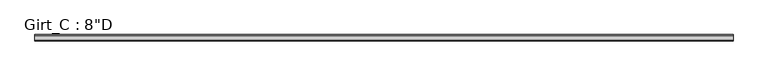
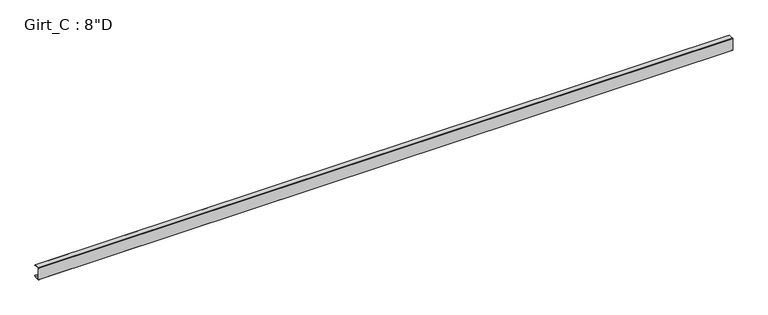
"""IFC4 building model written with IfcOpenShell, lengths in millimetres: beam geometry."""

import ifcopenshell
import ifcopenshell.guid

model = None  # the IFC model being written
_history = None  # IfcOwnerHistory: only IFC2X3 demands one
_inside = {}  # id of a spatial element -> (the spatial element, [elements in it])
_under = {}  # id of a project, library or spatial element -> (it, [spatial elements below it])
_declared = {}  # id of a project -> (the project, [libraries it declares])
_typed = {}  # id of a type object -> (the type object, [elements of that type])
_made_of = {}  # id of a material, layer set ... -> (it, [elements and type objects made of it])


def new_model(schema):
    """Start an empty IFC model of exactly this schema.

    Asked for "IFC4X3", IfcOpenShell would pick the latest addendum, in which some entities
    have other attributes; the version numbers below select the first issue.
    IFC2X3 requires an IfcOwnerHistory on every rooted entity: one is made here for all.
    """
    global model, _history
    if schema == "IFC4X3":
        model = ifcopenshell.file(schema_version=(4, 3, 0, 0))
    else:
        model = ifcopenshell.file(schema=schema)
    _inside.clear()
    _under.clear()
    _declared.clear()
    _typed.clear()
    _made_of.clear()
    _history = None
    if model.schema == "IFC2X3":
        org = make("IfcOrganization", Name="unknown")
        user = make(
            "IfcPersonAndOrganization",
            ThePerson=make("IfcPerson", FamilyName="unknown"),
            TheOrganization=org,
        )
        app = make(
            "IfcApplication",
            ApplicationDeveloper=org,
            Version="unknown",
            ApplicationFullName="unknown",
            ApplicationIdentifier="unknown",
        )
        _history = make(
            "IfcOwnerHistory",
            OwningUser=user,
            OwningApplication=app,
            ChangeAction="ADDED",
            CreationDate=0,
        )
    return model


def make(cls, **values):
    """One entity of the class cls with the attributes given. An attribute that is None is left unset."""
    return model.create_entity(
        cls, **{name: value for name, value in values.items() if value is not None}
    )


def rooted(cls, **values):
    """An entity with a GlobalId (a new one), such as an element, a storey or a relation."""
    return make(cls, GlobalId=ifcopenshell.guid.new(), OwnerHistory=_history, **values)


def si_unit(unit_type, name, prefix=None):
    """IfcSIUnit, for example si_unit("LENGTHUNIT", "METRE", prefix="MILLI")."""
    return make("IfcSIUnit", UnitType=unit_type, Prefix=prefix, Name=name)


def assignment(units):
    """IfcUnitAssignment: the units of a project."""
    return None if units is None else make("IfcUnitAssignment", Units=units)


def point(xyz):
    """IfcCartesianPoint."""
    return None if xyz is None else make("IfcCartesianPoint", Coordinates=xyz)


def direction(xyz):
    """IfcDirection."""
    return None if xyz is None else make("IfcDirection", DirectionRatios=xyz)


def frame(location, z_axis=None, x_axis=None):
    """IfcAxis2Placement3D, a coordinate frame: its origin and axes. An axis left out is left unset."""
    return make(
        "IfcAxis2Placement3D",
        Location=point(location),
        Axis=direction(z_axis),
        RefDirection=direction(x_axis),
    )


def frame_2d(location, x_axis=None):
    """IfcAxis2Placement2D, a coordinate frame in the plane: its origin and x axis."""
    return make(
        "IfcAxis2Placement2D", Location=point(location), RefDirection=direction(x_axis)
    )


def origin():
    """The frame at (0, 0, 0) with its axes left unset."""
    return frame((0.0, 0.0, 0.0))


def place(relative_to, where):
    """IfcLocalPlacement: puts the frame where relative to a parent placement (None: the world)."""
    return make(
        "IfcLocalPlacement", PlacementRelTo=relative_to, RelativePlacement=where
    )


def context(
    kind, dimensions, precision=None, world=None, true_north=None, identifier=None
):
    """IfcGeometricRepresentationContext, for example the 3D "Model" context."""
    return make(
        "IfcGeometricRepresentationContext",
        ContextIdentifier=identifier,
        ContextType=kind,
        CoordinateSpaceDimension=dimensions,
        Precision=precision,
        WorldCoordinateSystem=world,
        TrueNorth=true_north,
    )


def project(units=None, contexts=None):
    """IfcProject with its units and contexts."""
    return rooted(
        "IfcProject",
        Name="project",
        RepresentationContexts=contexts,
        UnitsInContext=assignment(units),
    )


def spatial(cls, under=None, at=None, **own):
    """A site, building, storey or space (cls), placed at a placement, below another one or the project."""
    s = rooted(cls, ObjectPlacement=at, **own)
    if under is not None:
        _under.setdefault(under.id(), (under, []))[1].append(s)
    return s


def polyline(points):
    """IfcPolyline through the points."""
    return make("IfcPolyline", Points=[point(p) for p in points])


def circle_curve(where, radius):
    """IfcCircle in the frame where."""
    return make("IfcCircle", Position=where, Radius=radius)


def trimmed(basis, trim1, trim2, sense, master):
    """IfcTrimmedCurve: the piece of a basis curve between two trims."""
    return make(
        "IfcTrimmedCurve",
        BasisCurve=basis,
        Trim1=trim1,
        Trim2=trim2,
        SenseAgreement=sense,
        MasterRepresentation=master,
    )


def segment(curve, same_sense, transition):
    """IfcCompositeCurveSegment."""
    return make(
        "IfcCompositeCurveSegment",
        Transition=transition,
        SameSense=same_sense,
        ParentCurve=curve,
    )


def composite_curve(segments, self_intersect=None):
    """IfcCompositeCurve: segments joined end to end."""
    return make("IfcCompositeCurve", Segments=segments, SelfIntersect=self_intersect)


def outline(outer, holes=None, kind="AREA"):
    """IfcArbitraryClosedProfileDef: a profile drawn as a closed curve; with holes, ...WithVoids."""
    if holes is None:
        return make("IfcArbitraryClosedProfileDef", ProfileType=kind, OuterCurve=outer)
    return make(
        "IfcArbitraryProfileDefWithVoids",
        ProfileType=kind,
        OuterCurve=outer,
        InnerCurves=holes,
    )


def extrude(swept, where, along, depth):
    """IfcExtrudedAreaSolid: the profile swept, set in the frame where, extruded along a direction by depth."""
    return make(
        "IfcExtrudedAreaSolid",
        SweptArea=swept,
        Position=where,
        ExtrudedDirection=direction(along),
        Depth=depth,
    )


def shape(context_of_items, identifier, shape_type, items):
    """IfcShapeRepresentation: the items that make up one representation, for example the "Body"."""
    return make(
        "IfcShapeRepresentation",
        ContextOfItems=context_of_items,
        RepresentationIdentifier=identifier,
        RepresentationType=shape_type,
        Items=items,
    )


def source(mapping_origin, context_of_items, identifier, shape_type, items):
    """IfcRepresentationMap: a shape defined once, which mapped items show again and again."""
    return make(
        "IfcRepresentationMap",
        MappingOrigin=mapping_origin,
        MappedRepresentation=shape(context_of_items, identifier, shape_type, items),
    )


def transform(
    local_origin,
    x_axis=None,
    y_axis=None,
    z_axis=None,
    scale=None,
    scale2=None,
    scale3=None,
    uniform=True,
):
    """IfcCartesianTransformationOperator3D, or its non-uniform kind. x_axis, y_axis, z_axis: its Axis1, 2, 3."""
    if uniform:
        return make(
            "IfcCartesianTransformationOperator3D",
            Axis1=direction(x_axis),
            Axis2=direction(y_axis),
            LocalOrigin=point(local_origin),
            Scale=scale,
            Axis3=direction(z_axis),
        )
    return make(
        "IfcCartesianTransformationOperator3DnonUniform",
        Axis1=direction(x_axis),
        Axis2=direction(y_axis),
        LocalOrigin=point(local_origin),
        Scale=scale,
        Axis3=direction(z_axis),
        Scale2=scale2,
        Scale3=scale3,
    )


def mapped(mapping_source, mapping_target):
    """IfcMappedItem: shows the shape of a source again, moved by a transform."""
    return make(
        "IfcMappedItem", MappingSource=mapping_source, MappingTarget=mapping_target
    )


def made_of(thing, what):
    """Note that an element or type object is made of a material, layer set ...; save() writes the relation."""
    if what is not None:
        _made_of.setdefault(what.id(), (what, []))[1].append(thing)
    return thing


def element(
    cls,
    number,
    at=None,
    inside=None,
    cuts=None,
    type_object=None,
    material=None,
    context=None,
    identifier="Body",
    shape_type=None,
    held_by="IfcProductDefinitionShape",
    body=None,
    shapes=None,
    **own,
):
    """One element of the class cls, such as IfcWall. Its Tag is "e" and its number.

    at: its placement. inside: the storey or other place that contains it. cuts: it is an
    opening in that element (IfcRelVoidsElement). A single representation is given by context,
    identifier, shape_type and body (its items); several are given by shapes. held_by: the class
    of the entity that holds the representations. save() writes the other relations.
    """
    e = rooted(cls, Tag="e%d" % number, ObjectPlacement=at, **own)
    if body is not None:
        shapes = [shape(context, identifier, shape_type, body)]
    if shapes is not None:
        e.Representation = make(held_by, Representations=shapes)
    if inside is not None:
        _inside.setdefault(inside.id(), (inside, []))[1].append(e)
    if cuts is not None:
        rooted(
            "IfcRelVoidsElement", RelatingBuildingElement=cuts, RelatedOpeningElement=e
        )
    if type_object is not None:
        _typed.setdefault(type_object.id(), (type_object, []))[1].append(e)
    return made_of(e, material)


def aggregate(whole, parts):
    """IfcRelAggregates: a whole, such as a stair, and the parts it consists of."""
    return rooted("IfcRelAggregates", RelatingObject=whole, RelatedObjects=parts)


def save(model, path):
    """Write the relations noted so far, then the file.

    IfcRelAggregates (storeys below a building ...), IfcRelContainedInSpatialStructure (elements
    in a storey), IfcRelDefinesByType, IfcRelAssociatesMaterial and IfcRelDeclares: one each for
    every whole, place, type object, material and project.
    """
    for whole, parts in _under.values():
        aggregate(whole, parts)
    for where, things in _inside.values():
        rooted(
            "IfcRelContainedInSpatialStructure",
            RelatedElements=things,
            RelatingStructure=where,
        )
    for kind, things in _typed.values():
        rooted("IfcRelDefinesByType", RelatedObjects=things, RelatingType=kind)
    for what, things in _made_of.values():
        rooted("IfcRelAssociatesMaterial", RelatedObjects=things, RelatingMaterial=what)
    for by, libraries in _declared.values():
        rooted("IfcRelDeclares", RelatingContext=by, RelatedDefinitions=libraries)
    model.write(path)


def beam_b678a68b(model_context):
    return source(origin(), model_context, "Body", "SweptSolid", [
        extrude(outline(composite_curve([segment(polyline([(87.5109375, 101.6), (99.7560415, 87.0068534), (97.6278742, 85.221109), (86.2154765, 98.821875), (3.3005807, 98.821875)]), True, "CONTINUOUS"), segment(trimmed(circle_curve(frame_2d((3.3741066, 96.8381931)), 1.9850441), [point((3.3005807, 98.821875))], [point((1.3890625, 96.8381931))], True, "CARTESIAN"), True, "CONTINUOUS"), segment(polyline([(1.3890625, 96.8381931), (1.3890625, -96.8389339)]), True, "CONTINUOUS"), segment(trimmed(circle_curve(frame_2d((3.3748024, -96.8389339)), 1.9857399), [point((1.3890625, -96.8389339))], [point((3.2694106, -98.821875))], True, "CARTESIAN"), True, "CONTINUOUS"), segment(polyline([(3.2694106, -98.821875), (86.2154765, -98.821875), (97.6510975, -85.1934327), (99.7792647, -86.979177), (87.5109375, -101.6), (3.3734375, -101.6)]), True, "CONTINUOUS"), segment(trimmed(circle_curve(frame_2d((3.3734375, -96.8375)), 4.7625), [point((3.3734375, -101.6))], [point((-1.3890625, -96.8375))], False, "CARTESIAN"), True, "CONTINUOUS"), segment(polyline([(-1.3890625, -96.8375), (-1.3890625, 96.8375)]), True, "CONTINUOUS"), segment(trimmed(circle_curve(frame_2d((3.3734375, 96.8375)), 4.7625), [point((-1.3890625, 96.8375))], [point((3.3734375, 101.6))], False, "CARTESIAN"), True, "CONTINUOUS"), segment(polyline([(3.3734375, 101.6), (87.5109375, 101.6)]), True, "CONTINUOUS")], self_intersect=False)), frame((-5654.675, 0.0, 0.0), z_axis=(1.0, 0.0, 0.0), x_axis=(0.0, 1.0, 0.0)), (0.0, 0.0, 1.0), 11309.35),
    ])


if __name__ == "__main__":
    model = new_model("IFC4")
    model_context = context("Model", 3, world=origin())
    ifc_project = project(units=[si_unit("LENGTHUNIT", "METRE", prefix="MILLI")], contexts=[model_context])
    site = spatial("IfcSite", under=ifc_project)
    building = spatial("IfcBuilding", under=site)
    placement = place(None, origin())
    beam_shape = beam_b678a68b(model_context)
    element("IfcBeam", 1, ObjectType="Girt_C : 8\"D", at=placement, inside=building, context=model_context, shape_type="MappedRepresentation", body=[
        mapped(beam_shape, transform((0.0, 0.0, 0.0), x_axis=(1.0, 0.0, 0.0), y_axis=(0.0, 1.0, 0.0), z_axis=(0.0, 0.0, 1.0))),
    ])
    save(model, "model.ifc")

# Revit data of these elements
# Type "Girt_C : 8\"D"
#   half leg = 0' - 1 3/4"
#   Web_Thickness = 0' - 0 7/64"
#   Length [instance default] = 10' - 0"
#   Leg_1 = 0' - 3 1/2"
#   Height = 0' - 8"
#   Structural Material [instance default] = none
# Element 1 (IfcBeam, "Girt_C : 8\"D")
#   Structural Material = GALVANIZED 'CEE' SECTION (8.0x3.5C - SEE STRUCT. DWGS)
#   Materials on its faces: "GALVANIZED 'CEE' SECTION (8.0x3.5C - SEE STRUCT. DWGS)"
# Materials
#   "GALVANIZED 'CEE' SECTION (8.0x3.5C - SEE STRUCT. DWGS)": class "Metal", colour RGB 137 146 153, transparency 0, Description = "Steel, mill finish", Cost = 0
